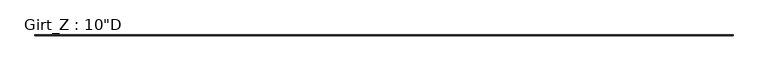
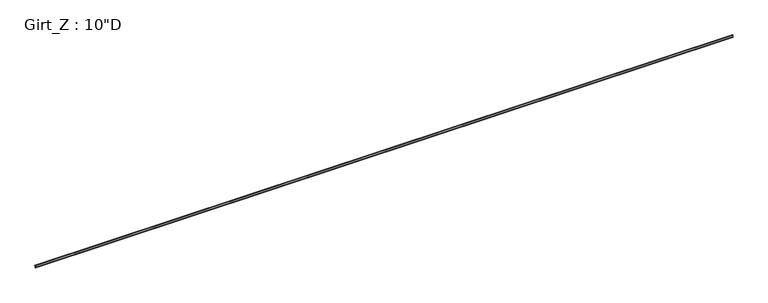
"""IFC4 building model written with IfcOpenShell, lengths in millimetres: beam geometry."""

import ifcopenshell
import ifcopenshell.guid

model = None  # the IFC model being written
_history = None  # IfcOwnerHistory: only IFC2X3 demands one
_inside = {}  # id of a spatial element -> (the spatial element, [elements in it])
_under = {}  # id of a project, library or spatial element -> (it, [spatial elements below it])
_declared = {}  # id of a project -> (the project, [libraries it declares])
_typed = {}  # id of a type object -> (the type object, [elements of that type])
_made_of = {}  # id of a material, layer set ... -> (it, [elements and type objects made of it])


def new_model(schema):
    """Start an empty IFC model of exactly this schema.

    Asked for "IFC4X3", IfcOpenShell would pick the latest addendum, in which some entities
    have other attributes; the version numbers below select the first issue.
    IFC2X3 requires an IfcOwnerHistory on every rooted entity: one is made here for all.
    """
    global model, _history
    if schema == "IFC4X3":
        model = ifcopenshell.file(schema_version=(4, 3, 0, 0))
    else:
        model = ifcopenshell.file(schema=schema)
    _inside.clear()
    _under.clear()
    _declared.clear()
    _typed.clear()
    _made_of.clear()
    _history = None
    if model.schema == "IFC2X3":
        org = make("IfcOrganization", Name="unknown")
        user = make(
            "IfcPersonAndOrganization",
            ThePerson=make("IfcPerson", FamilyName="unknown"),
            TheOrganization=org,
        )
        app = make(
            "IfcApplication",
            ApplicationDeveloper=org,
            Version="unknown",
            ApplicationFullName="unknown",
            ApplicationIdentifier="unknown",
        )
        _history = make(
            "IfcOwnerHistory",
            OwningUser=user,
            OwningApplication=app,
            ChangeAction="ADDED",
            CreationDate=0,
        )
    return model


def make(cls, **values):
    """One entity of the class cls with the attributes given. An attribute that is None is left unset."""
    return model.create_entity(
        cls, **{name: value for name, value in values.items() if value is not None}
    )


def rooted(cls, **values):
    """An entity with a GlobalId (a new one), such as an element, a storey or a relation."""
    return make(cls, GlobalId=ifcopenshell.guid.new(), OwnerHistory=_history, **values)


def si_unit(unit_type, name, prefix=None):
    """IfcSIUnit, for example si_unit("LENGTHUNIT", "METRE", prefix="MILLI")."""
    return make("IfcSIUnit", UnitType=unit_type, Prefix=prefix, Name=name)


def assignment(units):
    """IfcUnitAssignment: the units of a project."""
    return None if units is None else make("IfcUnitAssignment", Units=units)


def point(xyz):
    """IfcCartesianPoint."""
    return None if xyz is None else make("IfcCartesianPoint", Coordinates=xyz)


def direction(xyz):
    """IfcDirection."""
    return None if xyz is None else make("IfcDirection", DirectionRatios=xyz)


def frame(location, z_axis=None, x_axis=None):
    """IfcAxis2Placement3D, a coordinate frame: its origin and axes. An axis left out is left unset."""
    return make(
        "IfcAxis2Placement3D",
        Location=point(location),
        Axis=direction(z_axis),
        RefDirection=direction(x_axis),
    )


def frame_2d(location, x_axis=None):
    """IfcAxis2Placement2D, a coordinate frame in the plane: its origin and x axis."""
    return make(
        "IfcAxis2Placement2D", Location=point(location), RefDirection=direction(x_axis)
    )


def origin():
    """The frame at (0, 0, 0) with its axes left unset."""
    return frame((0.0, 0.0, 0.0))


def place(relative_to, where):
    """IfcLocalPlacement: puts the frame where relative to a parent placement (None: the world)."""
    return make(
        "IfcLocalPlacement", PlacementRelTo=relative_to, RelativePlacement=where
    )


def context(
    kind, dimensions, precision=None, world=None, true_north=None, identifier=None
):
    """IfcGeometricRepresentationContext, for example the 3D "Model" context."""
    return make(
        "IfcGeometricRepresentationContext",
        ContextIdentifier=identifier,
        ContextType=kind,
        CoordinateSpaceDimension=dimensions,
        Precision=precision,
        WorldCoordinateSystem=world,
        TrueNorth=true_north,
    )


def project(units=None, contexts=None):
    """IfcProject with its units and contexts."""
    return rooted(
        "IfcProject",
        Name="project",
        RepresentationContexts=contexts,
        UnitsInContext=assignment(units),
    )


def spatial(cls, under=None, at=None, **own):
    """A site, building, storey or space (cls), placed at a placement, below another one or the project."""
    s = rooted(cls, ObjectPlacement=at, **own)
    if under is not None:
        _under.setdefault(under.id(), (under, []))[1].append(s)
    return s


def polyline(points):
    """IfcPolyline through the points."""
    return make("IfcPolyline", Points=[point(p) for p in points])


def circle_curve(where, radius):
    """IfcCircle in the frame where."""
    return make("IfcCircle", Position=where, Radius=radius)


def trimmed(basis, trim1, trim2, sense, master):
    """IfcTrimmedCurve: the piece of a basis curve between two trims."""
    return make(
        "IfcTrimmedCurve",
        BasisCurve=basis,
        Trim1=trim1,
        Trim2=trim2,
        SenseAgreement=sense,
        MasterRepresentation=master,
    )


def segment(curve, same_sense, transition):
    """IfcCompositeCurveSegment."""
    return make(
        "IfcCompositeCurveSegment",
        Transition=transition,
        SameSense=same_sense,
        ParentCurve=curve,
    )


def composite_curve(segments, self_intersect=None):
    """IfcCompositeCurve: segments joined end to end."""
    return make("IfcCompositeCurve", Segments=segments, SelfIntersect=self_intersect)


def outline(outer, holes=None, kind="AREA"):
    """IfcArbitraryClosedProfileDef: a profile drawn as a closed curve; with holes, ...WithVoids."""
    if holes is None:
        return make("IfcArbitraryClosedProfileDef", ProfileType=kind, OuterCurve=outer)
    return make(
        "IfcArbitraryProfileDefWithVoids",
        ProfileType=kind,
        OuterCurve=outer,
        InnerCurves=holes,
    )


def extrude(swept, where, along, depth):
    """IfcExtrudedAreaSolid: the profile swept, set in the frame where, extruded along a direction by depth."""
    return make(
        "IfcExtrudedAreaSolid",
        SweptArea=swept,
        Position=where,
        ExtrudedDirection=direction(along),
        Depth=depth,
    )


def shape(context_of_items, identifier, shape_type, items):
    """IfcShapeRepresentation: the items that make up one representation, for example the "Body"."""
    return make(
        "IfcShapeRepresentation",
        ContextOfItems=context_of_items,
        RepresentationIdentifier=identifier,
        RepresentationType=shape_type,
        Items=items,
    )


def source(mapping_origin, context_of_items, identifier, shape_type, items):
    """IfcRepresentationMap: a shape defined once, which mapped items show again and again."""
    return make(
        "IfcRepresentationMap",
        MappingOrigin=mapping_origin,
        MappedRepresentation=shape(context_of_items, identifier, shape_type, items),
    )


def transform(
    local_origin,
    x_axis=None,
    y_axis=None,
    z_axis=None,
    scale=None,
    scale2=None,
    scale3=None,
    uniform=True,
):
    """IfcCartesianTransformationOperator3D, or its non-uniform kind. x_axis, y_axis, z_axis: its Axis1, 2, 3."""
    if uniform:
        return make(
            "IfcCartesianTransformationOperator3D",
            Axis1=direction(x_axis),
            Axis2=direction(y_axis),
            LocalOrigin=point(local_origin),
            Scale=scale,
            Axis3=direction(z_axis),
        )
    return make(
        "IfcCartesianTransformationOperator3DnonUniform",
        Axis1=direction(x_axis),
        Axis2=direction(y_axis),
        LocalOrigin=point(local_origin),
        Scale=scale,
        Axis3=direction(z_axis),
        Scale2=scale2,
        Scale3=scale3,
    )


def mapped(mapping_source, mapping_target):
    """IfcMappedItem: shows the shape of a source again, moved by a transform."""
    return make(
        "IfcMappedItem", MappingSource=mapping_source, MappingTarget=mapping_target
    )


def made_of(thing, what):
    """Note that an element or type object is made of a material, layer set ...; save() writes the relation."""
    if what is not None:
        _made_of.setdefault(what.id(), (what, []))[1].append(thing)
    return thing


def element(
    cls,
    number,
    at=None,
    inside=None,
    cuts=None,
    type_object=None,
    material=None,
    context=None,
    identifier="Body",
    shape_type=None,
    held_by="IfcProductDefinitionShape",
    body=None,
    shapes=None,
    **own,
):
    """One element of the class cls, such as IfcWall. Its Tag is "e" and its number.

    at: its placement. inside: the storey or other place that contains it. cuts: it is an
    opening in that element (IfcRelVoidsElement). A single representation is given by context,
    identifier, shape_type and body (its items); several are given by shapes. held_by: the class
    of the entity that holds the representations. save() writes the other relations.
    """
    e = rooted(cls, Tag="e%d" % number, ObjectPlacement=at, **own)
    if body is not None:
        shapes = [shape(context, identifier, shape_type, body)]
    if shapes is not None:
        e.Representation = make(held_by, Representations=shapes)
    if inside is not None:
        _inside.setdefault(inside.id(), (inside, []))[1].append(e)
    if cuts is not None:
        rooted(
            "IfcRelVoidsElement", RelatingBuildingElement=cuts, RelatedOpeningElement=e
        )
    if type_object is not None:
        _typed.setdefault(type_object.id(), (type_object, []))[1].append(e)
    return made_of(e, material)


def aggregate(whole, parts):
    """IfcRelAggregates: a whole, such as a stair, and the parts it consists of."""
    return rooted("IfcRelAggregates", RelatingObject=whole, RelatedObjects=parts)


def save(model, path):
    """Write the relations noted so far, then the file.

    IfcRelAggregates (storeys below a building ...), IfcRelContainedInSpatialStructure (elements
    in a storey), IfcRelDefinesByType, IfcRelAssociatesMaterial and IfcRelDeclares: one each for
    every whole, place, type object, material and project.
    """
    for whole, parts in _under.values():
        aggregate(whole, parts)
    for where, things in _inside.values():
        rooted(
            "IfcRelContainedInSpatialStructure",
            RelatedElements=things,
            RelatingStructure=where,
        )
    for kind, things in _typed.values():
        rooted("IfcRelDefinesByType", RelatedObjects=things, RelatingType=kind)
    for what, things in _made_of.values():
        rooted("IfcRelAssociatesMaterial", RelatedObjects=things, RelatingMaterial=what)
    for by, libraries in _declared.values():
        rooted("IfcRelDeclares", RelatingContext=by, RelatedDefinitions=libraries)
    model.write(path)


def beam_f2d5f719(model_context):
    return source(origin(), model_context, "Body", "SweptSolid", [
        extrude(outline(composite_curve([segment(polyline([(63.5, 127.0), (75.745104, 112.4068534), (73.6169367, 110.621109), (62.204539, 124.221875), (3.3005807, 124.221875)]), True, "CONTINUOUS"), segment(trimmed(circle_curve(frame_2d((3.3741066, 122.2381931)), 1.9850441), [point((3.3005807, 124.221875))], [point((1.3890625, 122.2381931))], True, "CARTESIAN"), True, "CONTINUOUS"), segment(polyline([(1.3890625, 122.2381931), (1.3890625, -122.2375)]), True, "CONTINUOUS"), segment(trimmed(circle_curve(frame_2d((-3.3734375, -122.2375)), 4.7625), [point((1.3890625, -122.2375))], [point((-3.3734375, -127.0))], False, "CARTESIAN"), True, "CONTINUOUS"), segment(polyline([(-3.3734375, -127.0), (-63.5, -127.0), (-75.745104, -112.4068534), (-73.6169367, -110.621109), (-62.204539, -124.221875), (-3.2694106, -124.221875)]), True, "CONTINUOUS"), segment(trimmed(circle_curve(frame_2d((-3.3748024, -122.2389339)), 1.9857399), [point((-3.2694106, -124.221875))], [point((-1.3890625, -122.2389339))], True, "CARTESIAN"), True, "CONTINUOUS"), segment(polyline([(-1.3890625, -122.2389339), (-1.3890625, 122.2375)]), True, "CONTINUOUS"), segment(trimmed(circle_curve(frame_2d((3.3734375, 122.2375)), 4.7625), [point((-1.3890625, 122.2375))], [point((3.3734375, 127.0))], False, "CARTESIAN"), True, "CONTINUOUS"), segment(polyline([(3.3734375, 127.0), (63.5, 127.0)]), True, "CONTINUOUS")], self_intersect=False)), frame((-51295.3, 0.0, 0.0), z_axis=(1.0, 0.0, 0.0), x_axis=(0.0, 1.0, 0.0)), (0.0, 0.0, 1.0), 102590.6),
    ])


if __name__ == "__main__":
    model = new_model("IFC4")
    model_context = context("Model", 3, world=origin())
    ifc_project = project(units=[si_unit("LENGTHUNIT", "METRE", prefix="MILLI")], contexts=[model_context])
    site = spatial("IfcSite", under=ifc_project)
    building = spatial("IfcBuilding", under=site)
    placement = place(None, origin())
    beam_shape = beam_f2d5f719(model_context)
    element("IfcBeam", 1, ObjectType="Girt_Z : 10\"D", at=placement, inside=building, context=model_context, shape_type="MappedRepresentation", body=[
        mapped(beam_shape, transform((0.0, 0.0, 0.0), x_axis=(1.0, 0.0, 0.0), y_axis=(0.0, 1.0, 0.0), z_axis=(0.0, 0.0, 1.0))),
    ])
    save(model, "model.ifc")

# Revit data of these elements
# Type "Girt_Z : 10\"D"
#   Web_Thickness = 0' - 0 7/64"
#   Length [instance default] = 10' - 0"
#   Leg_1 = 0' - 2 1/2"
#   Height = 0' - 10"
#   Structural Material [instance default] = none
